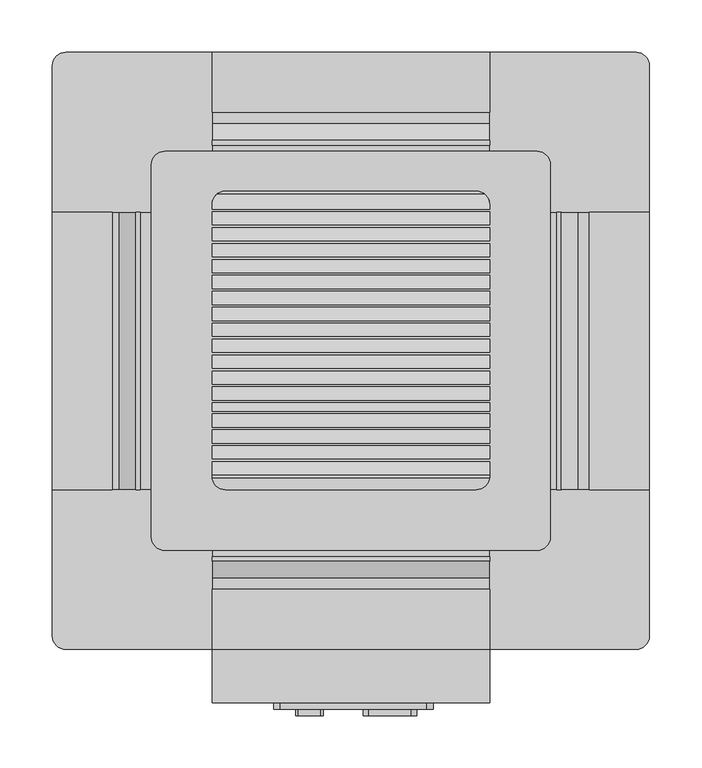
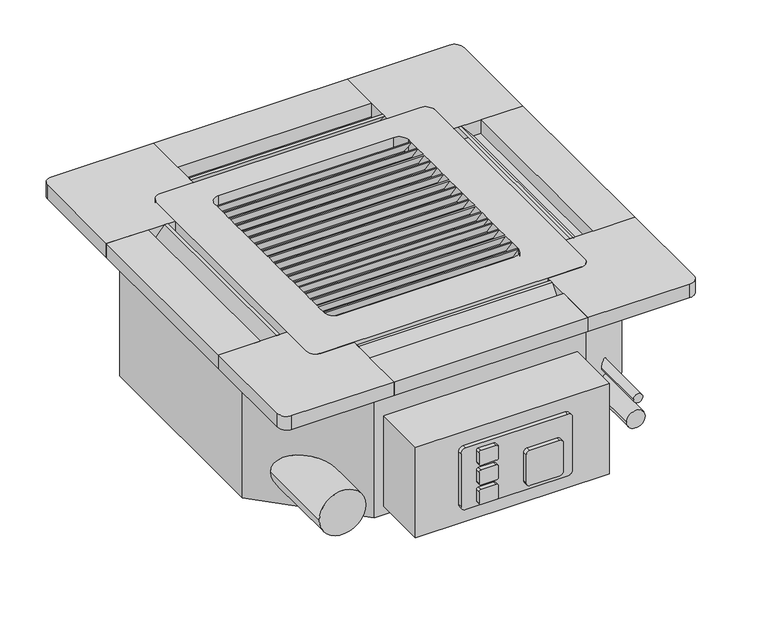
# IFC4 building model written with IfcOpenShell, lengths in millimetres: proxy geometry, PLFY-P-NCMU-E_4-way_24x24 : PLFY-P12NCMU-E.
# Revit data of these elements (continued)
# Type "PLFY-P-NCMU-E_4-way_24x24 : PLFY-P12NCMU-E"
#   Voltage Options = "208/230 VAC"
#   Unit Weight (LBS) = "37"
#   Subcategory = "HVAC"
#   Standard Air Filter = "Polypropylene Honeycomb"
#   Specification URL = "http://www.mrslim.com/customerCare/resources.asp"
#   Sound Pressure Levels (dB(A)) = "30-34-39"
#   SmartBIM Object Created BY = "Reed Construction Data"
#   Single Phase = "X"
#   Power Consumption Heating = "0.05 kW"
#   Power Consumption Cooling = "0.05 kW"
#   Model = "PLFY-P12NCMU-E"
#   Manufacturer URL = "http://www.mrslim.com/customerCare/resources.asp"
#   Manufacturer = "Mitsubishi Electric"
#   Installation URL = "http://www.mrslim.com/customerCare/resources.asp"
#   Heating Indoor = "70°F (21°C) DB, Outdoor 47°F (8°C) DB / 43°F (6°C) WB"
#   Grille Net Weight = "13 lbs. / 6 kg"
#   General FEATURES-10 = "i-see sensor option uses infrared rays to search for hot"
#   General FEATURES-09 = "Multiple sizes up to 36,000 Btu/h"
#   General FEATURES-08 = "Outside air capability"
#   General FEATURES-07 = "Built-in condensate lift mechanism; lifts to 33-1/2 in."
#   General FEATURES-06 = "Corner-pocket design for simplified installation"
#   General FEATURES-05 = "Four-speed fan settings and auto fan speed adjustment mode"
#   General FEATURES-04 = "Auto wave airflow in heating mode—unit independently"
#   General FEATURES-03 = "Customizable wide airflow pattern enables better air"
#   General FEATURES-02 = "Lightweight, low-profile compact design"
#   General FEATURES-01 = "R410A or R22 refrigerant-compatible"
#   Frequency = "60 Hz"
#   Flared Connection 2 = "1/2\""
#   Flared Connection 1 = "1/4\""
#   Fan capacity (CFM) = "280-320-350"
#   Fan Type*Quantity = "Turbo Fan x 1"
#   Fan Motor Type = "DC Motor"
#   Fan Motor Output = "0.050 kW"
#   Description = "Ceiling Recessed Units"
#   Current Heating = "0.23 A "
#   Current Cooling = "0.23 A "
#   Cooling Indoor = "80°F (27°C) DB / 67°F (19°C) WB, Outdoor 95°F (35°C) DB"
#   Assembly Code = "D3050200"
#   95 CSI = "15760"
#   04 CSI = "23 82 19"
#   (Option) i-see Sensor Corner Panel = "PAC-SA1ME-E"
#   (Option) Wireless Signal Receiver = "PAR-SA9FA-E"
#   (Option) Space Panel = "PAC-SH48AS-E"
#   (Option) Multi-function Casement = "PAC-SH53TM-E"
#   (Option) High-Efficiency Filter (MERV 10) = "AC-SH59KF-E"
#   (Option) Flange for Ventilation Air Intake = "PAC-SH65OF-E"
#   (Option) Air Outlet Shutter Plate (2 pieces) = "PAC-SH51SP-E"
#   Width = 1' - 10 7/16"
#   Voltage = 208 V
#   Unit Supply Air Flow [instance default] = 0 CFM
#   SmartBIM Object Version = 3
#   Refrigerant Pipe diameter (Liquid) = 0' - 0 1/4"
#   Refrigerant Pipe diameter (Gas) = 0' - 0 1/2"
#   Phase = 1
#   Nominal Heating Capacity = 13500.0 Btu/h
#   Nominal Cooling Capacity = 12000.0 Btu/h
#   Minimum Circuit Ampacity = 0.35 A
#   Maximum Overcurrent Protection = 15 A
#   Individual Supply Air Flow [instance default] = 0 CFM
#   Hertz = 60
#   Height = 0' - 8 3/16"
#   Fresh Air Intake Radius = 0' - 2 1/2"
#   Exhaust Air Flow [instance default] = 0 CFM
#   Emergency Drain Radius = 0' - 2 1/8"
#   Drain Pipe Radius = 0' - 1 1/4"
#   Drain Pipe Outer Radius = 0' - 1 3/8"
#   Depth = 1' - 10 7/16"
#   Default Elevation = 4' - 0"
#   D = 0' - 2 117/128"
#   Cut Out Hole Radius = 0' - 1 7/16"
#   Cut Out Hole Dia = 0' - 2 7/8"
#   C = 0' - 3 19/128"
#   Auto Vane Air Outlet Width = 0' - 2 1/4"
#   Auto Vane Air Outlet Length = 0' - 10"
#   Apparent Load = 0 VA
#   Air Inlet Width = 1' - 3"
#   Air Inlet Height = 1' - 3"
#   Sound Pressure Levels @ Mid Airflow (dBA) = 30
#   Sound Pressure Levels @ Low Airflow (dBA) = 34
#   Sound Pressure Levels @ High Airflow (dBA) = 39
#   Number of Poles = 2
#   Load Classification = HVAC
#   Grille Material = Paint White Cool Glossy
# Element 1 (IfcBuildingElementProxy, "PLFY-P-NCMU-E_4-way_24x24 : PLFY-P12NCMU-E")
#   Unit Supply Air Flow = 390 CFM
#   Individual Supply Air Flow = 97.5 CFM
#   Exhaust Air Flow = 20 CFM
#   Materials on its faces: "Paint White Cool Glossy"
# Materials
#   "Paint White Cool Glossy": class "Paint", colour RGB 242 242 255, transparency 0
